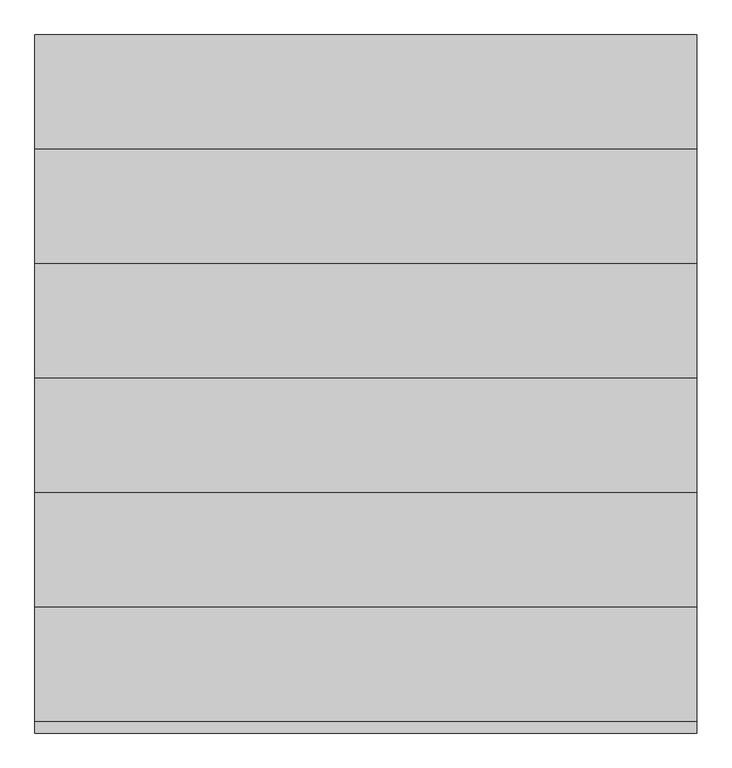
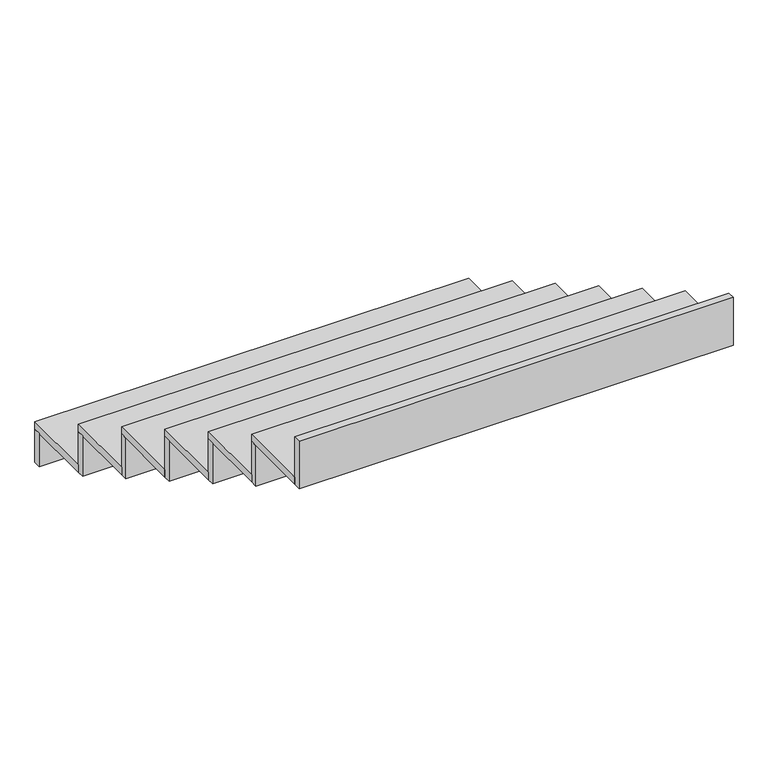
"""IFC4 building model written with IfcOpenShell, lengths in millimetres: stair flight geometry."""

from ifc_helpers import new_model, si_unit, frame, origin, place, context, project, spatial, polyline, outline, extrude, source, transform, mapped, element, save


def stair_flight_c018002c(model_context):
    return source(origin(), model_context, "Body", "SweptSolid", [
        extrude(outline(polyline([(52915.0, -2630.0), (52915.0, -2600.0), (54650.0, -2600.0), (54650.0, -2630.0), (52915.0, -2630.0)])), frame((0.0, 0.0, 18800.0), z_axis=(0.0, 0.0, 1.0), x_axis=(1.0, 0.0, 0.0)), (0.0, 0.0, 1.0), 141.4285714),
        extrude(outline(polyline([(54650.0, -2900.0), (52915.0, -2900.0), (52915.0, -2600.0), (54650.0, -2600.0), (54650.0, -2900.0)])), frame((0.0, 0.0, 18941.4285714), z_axis=(0.0, 0.0, 1.0), x_axis=(1.0, 0.0, 0.0)), (0.0, 0.0, 1.0), 30.0),
        extrude(outline(polyline([(52915.0, -2930.0), (52915.0, -2900.0), (54650.0, -2900.0), (54650.0, -2930.0), (52915.0, -2930.0)])), frame((0.0, 0.0, 18941.4285714), z_axis=(0.0, 0.0, 1.0), x_axis=(1.0, 0.0, 0.0)), (0.0, 0.0, 1.0), 171.4285714),
        extrude(outline(polyline([(54650.0, -3200.0), (52915.0, -3200.0), (52915.0, -2900.0), (54650.0, -2900.0), (54650.0, -3200.0)])), frame((0.0, 0.0, 19112.8571429), z_axis=(0.0, 0.0, 1.0), x_axis=(1.0, 0.0, 0.0)), (0.0, 0.0, 1.0), 30.0),
        extrude(outline(polyline([(52915.0, -3230.0), (52915.0, -3200.0), (54650.0, -3200.0), (54650.0, -3230.0), (52915.0, -3230.0)])), frame((0.0, 0.0, 19112.8571429), z_axis=(0.0, 0.0, 1.0), x_axis=(1.0, 0.0, 0.0)), (0.0, 0.0, 1.0), 171.4285714),
        extrude(outline(polyline([(54650.0, -3500.0), (52915.0, -3500.0), (52915.0, -3200.0), (54650.0, -3200.0), (54650.0, -3500.0)])), frame((0.0, 0.0, 19284.2857143), z_axis=(0.0, 0.0, 1.0), x_axis=(1.0, 0.0, 0.0)), (0.0, 0.0, 1.0), 30.0),
        extrude(outline(polyline([(52915.0, -3530.0), (52915.0, -3500.0), (54650.0, -3500.0), (54650.0, -3530.0), (52915.0, -3530.0)])), frame((0.0, 0.0, 19284.2857143), z_axis=(0.0, 0.0, 1.0), x_axis=(1.0, 0.0, 0.0)), (0.0, 0.0, 1.0), 171.4285714),
        extrude(outline(polyline([(54650.0, -3800.0), (52915.0, -3800.0), (52915.0, -3500.0), (54650.0, -3500.0), (54650.0, -3800.0)])), frame((0.0, 0.0, 19455.7142857), z_axis=(0.0, 0.0, 1.0), x_axis=(1.0, 0.0, 0.0)), (0.0, 0.0, 1.0), 30.0),
        extrude(outline(polyline([(52915.0, -3830.0), (52915.0, -3800.0), (54650.0, -3800.0), (54650.0, -3830.0), (52915.0, -3830.0)])), frame((0.0, 0.0, 19455.7142857), z_axis=(0.0, 0.0, 1.0), x_axis=(1.0, 0.0, 0.0)), (0.0, 0.0, 1.0), 171.4285714),
        extrude(outline(polyline([(54650.0, -4100.0), (52915.0, -4100.0), (52915.0, -3800.0), (54650.0, -3800.0), (54650.0, -4100.0)])), frame((0.0, 0.0, 19627.1428571), z_axis=(0.0, 0.0, 1.0), x_axis=(1.0, 0.0, 0.0)), (0.0, 0.0, 1.0), 30.0),
        extrude(outline(polyline([(52915.0, -4130.0), (52915.0, -4100.0), (54650.0, -4100.0), (54650.0, -4130.0), (52915.0, -4130.0)])), frame((0.0, 0.0, 19627.1428571), z_axis=(0.0, 0.0, 1.0), x_axis=(1.0, 0.0, 0.0)), (0.0, 0.0, 1.0), 171.4285714),
        extrude(outline(polyline([(54650.0, -4400.0), (52915.0, -4400.0), (52915.0, -4100.0), (54650.0, -4100.0), (54650.0, -4400.0)])), frame((0.0, 0.0, 19798.5714286), z_axis=(0.0, 0.0, 1.0), x_axis=(1.0, 0.0, 0.0)), (0.0, 0.0, 1.0), 30.0),
        extrude(outline(polyline([(52915.0, -4430.0), (52915.0, -4400.0), (54650.0, -4400.0), (54650.0, -4430.0), (52915.0, -4430.0)])), frame((0.0, 0.0, 19798.5714286), z_axis=(0.0, 0.0, 1.0), x_axis=(1.0, 0.0, 0.0)), (0.0, 0.0, 1.0), 201.4285714),
    ])


if __name__ == "__main__":
    model = new_model("IFC4")
    model_context = context("Model", 3, world=origin())
    ifc_project = project(units=[si_unit("LENGTHUNIT", "METRE", prefix="MILLI")], contexts=[model_context])
    site = spatial("IfcSite", under=ifc_project)
    building = spatial("IfcBuilding", under=site)
    placement = place(None, origin())
    stair_flight_shape = stair_flight_c018002c(model_context)
    element("IfcStairFlight", 1, at=placement, inside=building, context=model_context, shape_type="MappedRepresentation", body=[
        mapped(stair_flight_shape, transform((0.0, 0.0, 0.0), x_axis=(1.0, 0.0, 0.0), y_axis=(0.0, 1.0, 0.0), z_axis=(0.0, 0.0, 1.0))),
    ])
    save(model, "model.ifc")

# Revit data of these elements
# Element 1 (IfcStairFlight)
#   Materials on its faces: "00_Finish_Deco Tile"
# Materials
#   "00_Finish_Deco Tile": class "Finish", colour RGB 245 245 245, transparency 0, Description = "Ceramic Tile", Cost = 0
